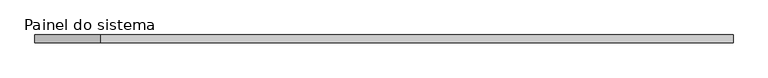
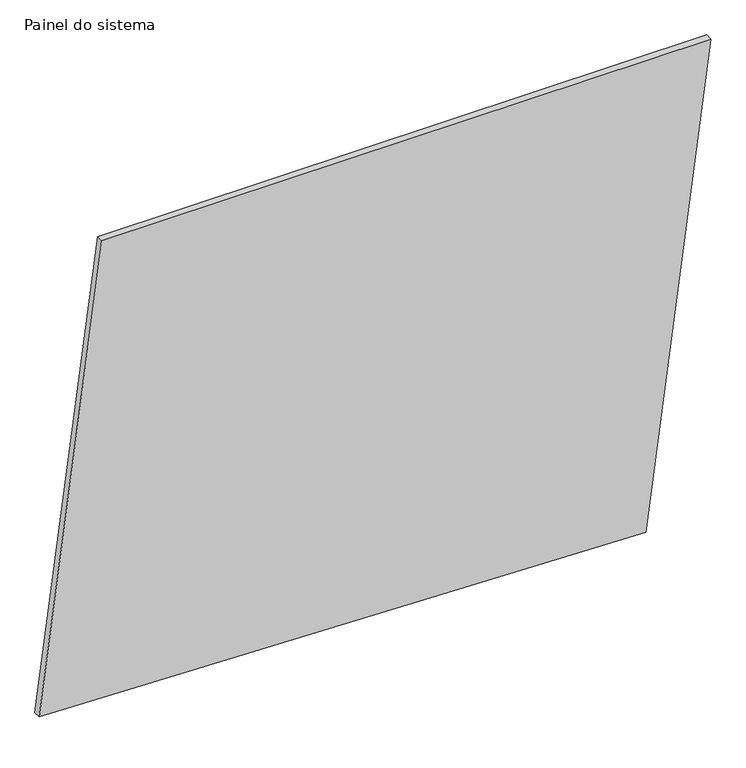
"""IFC4 building model written with IfcOpenShell, lengths in millimetres: plate geometry, Painel do sistema : Envidraçado."""

from ifc_helpers import new_model, si_unit, frame, origin, place, context, project, spatial, polyline, outline, extrude, source, transform, mapped, element, save


def painel_do_sistema_bb0fef57(model_context):
    return source(origin(), model_context, "Body", "SweptSolid", [
        extrude(outline(polyline([(59.0754793, -1146.9077135), (0.0, 924.746078), (1700.8197114, 1146.9077135), (1700.8197114, -932.4625368), (59.0754793, -1146.9077135)])), frame((0.0, 24.5, 0.0), z_axis=(0.0, 1.0, 0.0), x_axis=(0.0, 0.0, 1.0)), (0.0, 0.0, 1.0), 25.0),
    ])


if __name__ == "__main__":
    model = new_model("IFC4")
    model_context = context("Model", 3, world=origin())
    ifc_project = project(units=[si_unit("LENGTHUNIT", "METRE", prefix="MILLI")], contexts=[model_context])
    site = spatial("IfcSite", under=ifc_project)
    building = spatial("IfcBuilding", under=site)
    placement = place(None, origin())
    painel_do_sistema_shape = painel_do_sistema_bb0fef57(model_context)
    element("IfcPlate", 1, ObjectType="Painel do sistema : Envidraçado", at=placement, inside=building, context=model_context, shape_type="MappedRepresentation", body=[
        mapped(painel_do_sistema_shape, transform((0.0, 0.0, 0.0), x_axis=(1.0, 0.0, 0.0), y_axis=(0.0, 1.0, 0.0), z_axis=(0.0, 0.0, 1.0))),
    ])
    save(model, "model.ifc")

# Revit data of these elements
# Type "Painel do sistema : Envidraçado"
#   Construction Type Id = "GSP4R"
#   Analytic Construction = "Vidraça única Pilkington 1/8 pol"
#   Visual Light Transmittance = 0.9
#   Solar Heat Gain Coefficient = 0.86
#   Heat Transfer Coefficient (U) = 6.7069 W/(m²·K)
# Element 1 (IfcPlate, "Painel do sistema : Envidraçado")
#   Materials on its faces: "Vidro"
# Materials
#   "Vidro": class "Vidro", colour RGB 0 128 192, transparency 0.9, Description = "Vidro de sílica", Cost = 0
